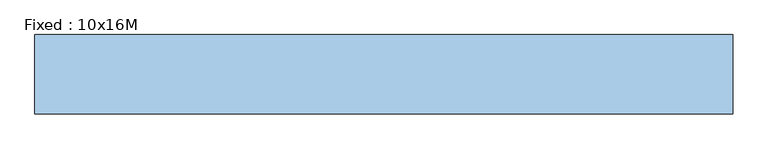
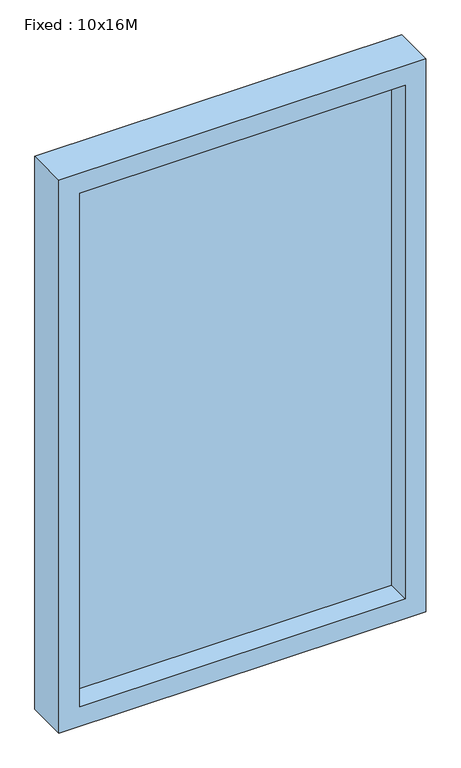
"""IFC4 building model written with IfcOpenShell, lengths in millimetres: window geometry, Fixed : 10x16M."""

import ifcopenshell
import ifcopenshell.guid

model = None  # the IFC model being written
_history = None  # IfcOwnerHistory: only IFC2X3 demands one
_inside = {}  # id of a spatial element -> (the spatial element, [elements in it])
_under = {}  # id of a project, library or spatial element -> (it, [spatial elements below it])
_declared = {}  # id of a project -> (the project, [libraries it declares])
_typed = {}  # id of a type object -> (the type object, [elements of that type])
_made_of = {}  # id of a material, layer set ... -> (it, [elements and type objects made of it])


def new_model(schema):
    """Start an empty IFC model of exactly this schema.

    Asked for "IFC4X3", IfcOpenShell would pick the latest addendum, in which some entities
    have other attributes; the version numbers below select the first issue.
    IFC2X3 requires an IfcOwnerHistory on every rooted entity: one is made here for all.
    """
    global model, _history
    if schema == "IFC4X3":
        model = ifcopenshell.file(schema_version=(4, 3, 0, 0))
    else:
        model = ifcopenshell.file(schema=schema)
    _inside.clear()
    _under.clear()
    _declared.clear()
    _typed.clear()
    _made_of.clear()
    _history = None
    if model.schema == "IFC2X3":
        org = make("IfcOrganization", Name="unknown")
        user = make(
            "IfcPersonAndOrganization",
            ThePerson=make("IfcPerson", FamilyName="unknown"),
            TheOrganization=org,
        )
        app = make(
            "IfcApplication",
            ApplicationDeveloper=org,
            Version="unknown",
            ApplicationFullName="unknown",
            ApplicationIdentifier="unknown",
        )
        _history = make(
            "IfcOwnerHistory",
            OwningUser=user,
            OwningApplication=app,
            ChangeAction="ADDED",
            CreationDate=0,
        )
    return model


def make(cls, **values):
    """One entity of the class cls with the attributes given. An attribute that is None is left unset."""
    return model.create_entity(
        cls, **{name: value for name, value in values.items() if value is not None}
    )


def rooted(cls, **values):
    """An entity with a GlobalId (a new one), such as an element, a storey or a relation."""
    return make(cls, GlobalId=ifcopenshell.guid.new(), OwnerHistory=_history, **values)


def si_unit(unit_type, name, prefix=None):
    """IfcSIUnit, for example si_unit("LENGTHUNIT", "METRE", prefix="MILLI")."""
    return make("IfcSIUnit", UnitType=unit_type, Prefix=prefix, Name=name)


def assignment(units):
    """IfcUnitAssignment: the units of a project."""
    return None if units is None else make("IfcUnitAssignment", Units=units)


def point(xyz):
    """IfcCartesianPoint."""
    return None if xyz is None else make("IfcCartesianPoint", Coordinates=xyz)


def direction(xyz):
    """IfcDirection."""
    return None if xyz is None else make("IfcDirection", DirectionRatios=xyz)


def frame(location, z_axis=None, x_axis=None):
    """IfcAxis2Placement3D, a coordinate frame: its origin and axes. An axis left out is left unset."""
    return make(
        "IfcAxis2Placement3D",
        Location=point(location),
        Axis=direction(z_axis),
        RefDirection=direction(x_axis),
    )


def origin():
    """The frame at (0, 0, 0) with its axes left unset."""
    return frame((0.0, 0.0, 0.0))


def place(relative_to, where):
    """IfcLocalPlacement: puts the frame where relative to a parent placement (None: the world)."""
    return make(
        "IfcLocalPlacement", PlacementRelTo=relative_to, RelativePlacement=where
    )


def context(
    kind, dimensions, precision=None, world=None, true_north=None, identifier=None
):
    """IfcGeometricRepresentationContext, for example the 3D "Model" context."""
    return make(
        "IfcGeometricRepresentationContext",
        ContextIdentifier=identifier,
        ContextType=kind,
        CoordinateSpaceDimension=dimensions,
        Precision=precision,
        WorldCoordinateSystem=world,
        TrueNorth=true_north,
    )


def project(units=None, contexts=None):
    """IfcProject with its units and contexts."""
    return rooted(
        "IfcProject",
        Name="project",
        RepresentationContexts=contexts,
        UnitsInContext=assignment(units),
    )


def spatial(cls, under=None, at=None, **own):
    """A site, building, storey or space (cls), placed at a placement, below another one or the project."""
    s = rooted(cls, ObjectPlacement=at, **own)
    if under is not None:
        _under.setdefault(under.id(), (under, []))[1].append(s)
    return s


def polyline(points):
    """IfcPolyline through the points."""
    return make("IfcPolyline", Points=[point(p) for p in points])


def outline(outer, holes=None, kind="AREA"):
    """IfcArbitraryClosedProfileDef: a profile drawn as a closed curve; with holes, ...WithVoids."""
    if holes is None:
        return make("IfcArbitraryClosedProfileDef", ProfileType=kind, OuterCurve=outer)
    return make(
        "IfcArbitraryProfileDefWithVoids",
        ProfileType=kind,
        OuterCurve=outer,
        InnerCurves=holes,
    )


def extrude(swept, where, along, depth):
    """IfcExtrudedAreaSolid: the profile swept, set in the frame where, extruded along a direction by depth."""
    return make(
        "IfcExtrudedAreaSolid",
        SweptArea=swept,
        Position=where,
        ExtrudedDirection=direction(along),
        Depth=depth,
    )


def shape(context_of_items, identifier, shape_type, items):
    """IfcShapeRepresentation: the items that make up one representation, for example the "Body"."""
    return make(
        "IfcShapeRepresentation",
        ContextOfItems=context_of_items,
        RepresentationIdentifier=identifier,
        RepresentationType=shape_type,
        Items=items,
    )


def source(mapping_origin, context_of_items, identifier, shape_type, items):
    """IfcRepresentationMap: a shape defined once, which mapped items show again and again."""
    return make(
        "IfcRepresentationMap",
        MappingOrigin=mapping_origin,
        MappedRepresentation=shape(context_of_items, identifier, shape_type, items),
    )


def transform(
    local_origin,
    x_axis=None,
    y_axis=None,
    z_axis=None,
    scale=None,
    scale2=None,
    scale3=None,
    uniform=True,
):
    """IfcCartesianTransformationOperator3D, or its non-uniform kind. x_axis, y_axis, z_axis: its Axis1, 2, 3."""
    if uniform:
        return make(
            "IfcCartesianTransformationOperator3D",
            Axis1=direction(x_axis),
            Axis2=direction(y_axis),
            LocalOrigin=point(local_origin),
            Scale=scale,
            Axis3=direction(z_axis),
        )
    return make(
        "IfcCartesianTransformationOperator3DnonUniform",
        Axis1=direction(x_axis),
        Axis2=direction(y_axis),
        LocalOrigin=point(local_origin),
        Scale=scale,
        Axis3=direction(z_axis),
        Scale2=scale2,
        Scale3=scale3,
    )


def mapped(mapping_source, mapping_target):
    """IfcMappedItem: shows the shape of a source again, moved by a transform."""
    return make(
        "IfcMappedItem", MappingSource=mapping_source, MappingTarget=mapping_target
    )


def made_of(thing, what):
    """Note that an element or type object is made of a material, layer set ...; save() writes the relation."""
    if what is not None:
        _made_of.setdefault(what.id(), (what, []))[1].append(thing)
    return thing


def element(
    cls,
    number,
    at=None,
    inside=None,
    cuts=None,
    type_object=None,
    material=None,
    context=None,
    identifier="Body",
    shape_type=None,
    held_by="IfcProductDefinitionShape",
    body=None,
    shapes=None,
    **own,
):
    """One element of the class cls, such as IfcWall. Its Tag is "e" and its number.

    at: its placement. inside: the storey or other place that contains it. cuts: it is an
    opening in that element (IfcRelVoidsElement). A single representation is given by context,
    identifier, shape_type and body (its items); several are given by shapes. held_by: the class
    of the entity that holds the representations. save() writes the other relations.
    """
    e = rooted(cls, Tag="e%d" % number, ObjectPlacement=at, **own)
    if body is not None:
        shapes = [shape(context, identifier, shape_type, body)]
    if shapes is not None:
        e.Representation = make(held_by, Representations=shapes)
    if inside is not None:
        _inside.setdefault(inside.id(), (inside, []))[1].append(e)
    if cuts is not None:
        rooted(
            "IfcRelVoidsElement", RelatingBuildingElement=cuts, RelatedOpeningElement=e
        )
    if type_object is not None:
        _typed.setdefault(type_object.id(), (type_object, []))[1].append(e)
    return made_of(e, material)


def aggregate(whole, parts):
    """IfcRelAggregates: a whole, such as a stair, and the parts it consists of."""
    return rooted("IfcRelAggregates", RelatingObject=whole, RelatedObjects=parts)


def save(model, path):
    """Write the relations noted so far, then the file.

    IfcRelAggregates (storeys below a building ...), IfcRelContainedInSpatialStructure (elements
    in a storey), IfcRelDefinesByType, IfcRelAssociatesMaterial and IfcRelDeclares: one each for
    every whole, place, type object, material and project.
    """
    for whole, parts in _under.values():
        aggregate(whole, parts)
    for where, things in _inside.values():
        rooted(
            "IfcRelContainedInSpatialStructure",
            RelatedElements=things,
            RelatingStructure=where,
        )
    for kind, things in _typed.values():
        rooted("IfcRelDefinesByType", RelatedObjects=things, RelatingType=kind)
    for what, things in _made_of.values():
        rooted("IfcRelAssociatesMaterial", RelatedObjects=things, RelatingMaterial=what)
    for by, libraries in _declared.values():
        rooted("IfcRelDeclares", RelatingContext=by, RelatedDefinitions=libraries)
    model.write(path)


def fixed_10x16m_885135a8(model_context):
    return source(origin(), model_context, "Body", "SweptSolid", [
        extrude(outline(polyline([(2412.0, 506.0), (2412.0, -506.0), (800.0, -506.0), (800.0, 506.0), (2412.0, 506.0)]), holes=[polyline([(857.0, 449.0), (857.0, -449.0), (2355.0, -449.0), (2355.0, 449.0), (857.0, 449.0)])]), frame((0.0, 69.0, 0.0), z_axis=(0.0, 1.0, 0.0), x_axis=(0.0, 0.0, 1.0)), (0.0, 0.0, 1.0), 115.0),
        extrude(outline(polyline([(-449.0, 162.0), (449.0, 162.0), (449.0, 134.0), (-449.0, 134.0), (-449.0, 162.0)])), frame((0.0, 0.0, 857.0), z_axis=(0.0, 0.0, 1.0), x_axis=(1.0, 0.0, 0.0)), (0.0, 0.0, 1.0), 1498.0),
    ])


if __name__ == "__main__":
    model = new_model("IFC4")
    model_context = context("Model", 3, world=origin())
    ifc_project = project(units=[si_unit("LENGTHUNIT", "METRE", prefix="MILLI")], contexts=[model_context])
    site = spatial("IfcSite", under=ifc_project)
    building = spatial("IfcBuilding", under=site)
    placement = place(None, origin())
    fixed_10x16m_shape = fixed_10x16m_885135a8(model_context)
    element("IfcWindow", 1, ObjectType="Fixed : 10x16M", at=placement, inside=building, context=model_context, shape_type="MappedRepresentation", body=[
        mapped(fixed_10x16m_shape, transform((0.0, 0.0, 0.0), x_axis=(1.0, 0.0, 0.0), y_axis=(0.0, 1.0, 0.0), z_axis=(0.0, 0.0, 1.0))),
    ])
    save(model, "model.ifc")

# Revit data of these elements
# Type "Fixed : 10x16M"
#   Type Mark = "59"
#   Creator Organization [instance default] = "© Danish Educational Content"
#   Creator Name [instance default] = "© Erik Falck Jørgensen"
#   Creator Build [instance default] = "2017.0801.0"
#   Analytic Construction = "<None>"
#   length#5 = -22 mm
#   length#4 = -50 mm
#   length#3 = 100 mm
#   length#2 = 57 mm
#   length#1 = 0 mm
#   Seal Width = 12 mm
#   Rough Width = 1012 mm
#   Rough Height = 1612 mm
#   Rebate Depth = 50 mm
#   Height = 1588 mm
#   Glass Thickness = 28 mm
#   Exterior Direction [instance default] = 0.00°
#   Default Sill Height = 800 mm
#   Width = 988 mm
#   Case Width = 45 mm
#   Case Depth = 115 mm
#   Sealing = no
#   Wall Closure = 1
#   Above Cutplane [instance default] = no
#   Wall Surface = none
#   Sill Plate = none
#   Glass = none
#   Embrasure = none
#   Case/Transom = none
#   Assembly Code = ""
# Element 1 (IfcWindow, "Fixed : 10x16M")
#   Materials on its faces: "Default Frame/Mullion (Interior/Exterior)", "Glass"
# Materials
#   "Default Frame/Mullion (Interior/Exterior)": class "Generic", colour RGB 205 205 205, transparency 0, Description = "Udefineret karm/ramme materiale", Cost = 0
#   "Glass": class "Glass", colour RGB 180 200 255, transparency 0.75, Description = "Generisk glas", Cost = 0
